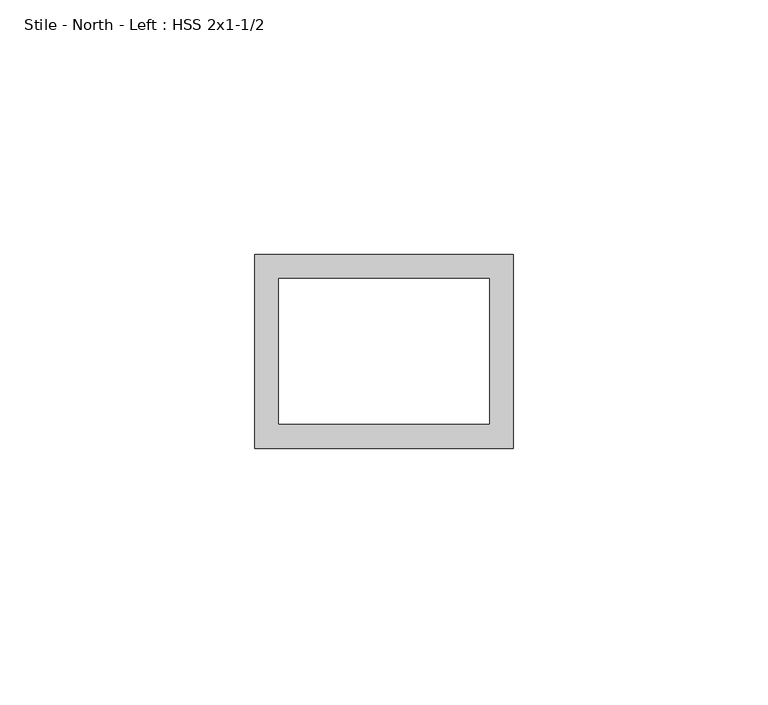
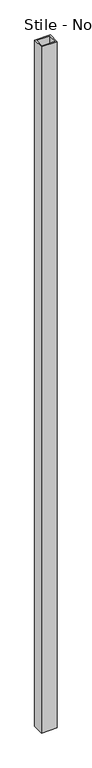
"""IFC4 building model written with IfcOpenShell, lengths in millimetres: proxy geometry, Stile - North - Left : HSS 2x1-1/2."""

from ifc_helpers import new_model, si_unit, frame, origin, place, context, project, spatial, polyline, outline, extrude, source, transform, mapped, element, save


def stile_north_left_hss_2x1_1_2_25622c15(model_context):
    return source(origin(), model_context, "Body", "SweptSolid", [
        extrude(outline(polyline([(587365.8934739, -531785.2663841), (587416.6934739, -531785.2663841), (587416.6934739, -531823.3663841), (587365.8934739, -531823.3663841), (587365.8934739, -531785.2663841)]), holes=[polyline([(587370.6559739, -531790.0288841), (587370.6559739, -531818.6038841), (587411.9309739, -531818.6038841), (587411.9309739, -531790.0288841), (587370.6559739, -531790.0288841)])]), frame((0.0, 0.0, 50.8), z_axis=(0.0, 0.0, 1.0), x_axis=(1.0, 0.0, 0.0)), (0.0, 0.0, 1.0), 2349.5),
    ])


if __name__ == "__main__":
    model = new_model("IFC4")
    model_context = context("Model", 3, world=origin())
    ifc_project = project(units=[si_unit("LENGTHUNIT", "METRE", prefix="MILLI")], contexts=[model_context])
    site = spatial("IfcSite", under=ifc_project)
    building = spatial("IfcBuilding", under=site)
    placement = place(None, origin())
    stile_north_left_hss_2x1_1_2_shape = stile_north_left_hss_2x1_1_2_25622c15(model_context)
    element("IfcBuildingElementProxy", 1, Name="Stile - North - Left : HSS 2x1-1/2", ObjectType="Stile - North - Left : HSS 2x1-1/2", at=placement, inside=building, context=model_context, shape_type="MappedRepresentation", body=[
        mapped(stile_north_left_hss_2x1_1_2_shape, transform((0.0, 0.0, 0.0), x_axis=(1.0, 0.0, 0.0), y_axis=(0.0, 1.0, 0.0), z_axis=(0.0, 0.0, 1.0))),
    ])
    save(model, "model.ifc")

# Revit data of these elements
# Element 1 (IfcBuildingElementProxy, "Stile - North - Left : HSS 2x1-1/2")
#   Materials on its faces: "1-1/2\"X2\" GALV. STL HSS TUBING"
# Materials
#   "1-1/2\"X2\" GALV. STL HSS TUBING": class "Generic", colour RGB 211 211 207, transparency 0, Cost = 0
